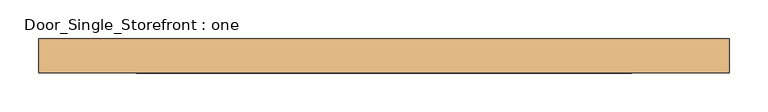
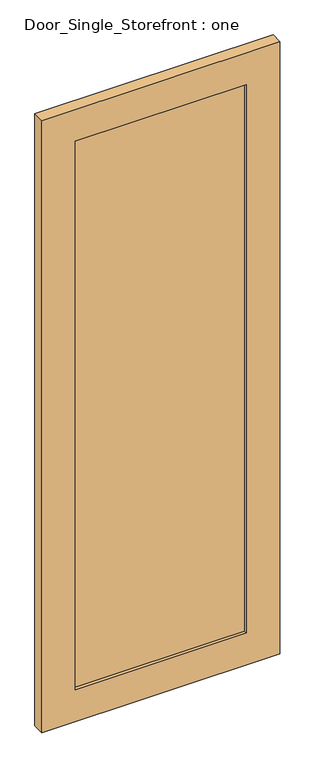
"""IFC4 building model written with IfcOpenShell, lengths in millimetres: door geometry, Door_Single_Storefront : one."""

import ifcopenshell
import ifcopenshell.guid

model = None  # the IFC model being written
_history = None  # IfcOwnerHistory: only IFC2X3 demands one
_inside = {}  # id of a spatial element -> (the spatial element, [elements in it])
_under = {}  # id of a project, library or spatial element -> (it, [spatial elements below it])
_declared = {}  # id of a project -> (the project, [libraries it declares])
_typed = {}  # id of a type object -> (the type object, [elements of that type])
_made_of = {}  # id of a material, layer set ... -> (it, [elements and type objects made of it])


def new_model(schema):
    """Start an empty IFC model of exactly this schema.

    Asked for "IFC4X3", IfcOpenShell would pick the latest addendum, in which some entities
    have other attributes; the version numbers below select the first issue.
    IFC2X3 requires an IfcOwnerHistory on every rooted entity: one is made here for all.
    """
    global model, _history
    if schema == "IFC4X3":
        model = ifcopenshell.file(schema_version=(4, 3, 0, 0))
    else:
        model = ifcopenshell.file(schema=schema)
    _inside.clear()
    _under.clear()
    _declared.clear()
    _typed.clear()
    _made_of.clear()
    _history = None
    if model.schema == "IFC2X3":
        org = make("IfcOrganization", Name="unknown")
        user = make(
            "IfcPersonAndOrganization",
            ThePerson=make("IfcPerson", FamilyName="unknown"),
            TheOrganization=org,
        )
        app = make(
            "IfcApplication",
            ApplicationDeveloper=org,
            Version="unknown",
            ApplicationFullName="unknown",
            ApplicationIdentifier="unknown",
        )
        _history = make(
            "IfcOwnerHistory",
            OwningUser=user,
            OwningApplication=app,
            ChangeAction="ADDED",
            CreationDate=0,
        )
    return model


def make(cls, **values):
    """One entity of the class cls with the attributes given. An attribute that is None is left unset."""
    return model.create_entity(
        cls, **{name: value for name, value in values.items() if value is not None}
    )


def rooted(cls, **values):
    """An entity with a GlobalId (a new one), such as an element, a storey or a relation."""
    return make(cls, GlobalId=ifcopenshell.guid.new(), OwnerHistory=_history, **values)


def si_unit(unit_type, name, prefix=None):
    """IfcSIUnit, for example si_unit("LENGTHUNIT", "METRE", prefix="MILLI")."""
    return make("IfcSIUnit", UnitType=unit_type, Prefix=prefix, Name=name)


def assignment(units):
    """IfcUnitAssignment: the units of a project."""
    return None if units is None else make("IfcUnitAssignment", Units=units)


def point(xyz):
    """IfcCartesianPoint."""
    return None if xyz is None else make("IfcCartesianPoint", Coordinates=xyz)


def direction(xyz):
    """IfcDirection."""
    return None if xyz is None else make("IfcDirection", DirectionRatios=xyz)


def frame(location, z_axis=None, x_axis=None):
    """IfcAxis2Placement3D, a coordinate frame: its origin and axes. An axis left out is left unset."""
    return make(
        "IfcAxis2Placement3D",
        Location=point(location),
        Axis=direction(z_axis),
        RefDirection=direction(x_axis),
    )


def origin():
    """The frame at (0, 0, 0) with its axes left unset."""
    return frame((0.0, 0.0, 0.0))


def place(relative_to, where):
    """IfcLocalPlacement: puts the frame where relative to a parent placement (None: the world)."""
    return make(
        "IfcLocalPlacement", PlacementRelTo=relative_to, RelativePlacement=where
    )


def context(
    kind, dimensions, precision=None, world=None, true_north=None, identifier=None
):
    """IfcGeometricRepresentationContext, for example the 3D "Model" context."""
    return make(
        "IfcGeometricRepresentationContext",
        ContextIdentifier=identifier,
        ContextType=kind,
        CoordinateSpaceDimension=dimensions,
        Precision=precision,
        WorldCoordinateSystem=world,
        TrueNorth=true_north,
    )


def project(units=None, contexts=None):
    """IfcProject with its units and contexts."""
    return rooted(
        "IfcProject",
        Name="project",
        RepresentationContexts=contexts,
        UnitsInContext=assignment(units),
    )


def spatial(cls, under=None, at=None, **own):
    """A site, building, storey or space (cls), placed at a placement, below another one or the project."""
    s = rooted(cls, ObjectPlacement=at, **own)
    if under is not None:
        _under.setdefault(under.id(), (under, []))[1].append(s)
    return s


def polyline(points):
    """IfcPolyline through the points."""
    return make("IfcPolyline", Points=[point(p) for p in points])


def outline(outer, holes=None, kind="AREA"):
    """IfcArbitraryClosedProfileDef: a profile drawn as a closed curve; with holes, ...WithVoids."""
    if holes is None:
        return make("IfcArbitraryClosedProfileDef", ProfileType=kind, OuterCurve=outer)
    return make(
        "IfcArbitraryProfileDefWithVoids",
        ProfileType=kind,
        OuterCurve=outer,
        InnerCurves=holes,
    )


def extrude(swept, where, along, depth):
    """IfcExtrudedAreaSolid: the profile swept, set in the frame where, extruded along a direction by depth."""
    return make(
        "IfcExtrudedAreaSolid",
        SweptArea=swept,
        Position=where,
        ExtrudedDirection=direction(along),
        Depth=depth,
    )


def shape(context_of_items, identifier, shape_type, items):
    """IfcShapeRepresentation: the items that make up one representation, for example the "Body"."""
    return make(
        "IfcShapeRepresentation",
        ContextOfItems=context_of_items,
        RepresentationIdentifier=identifier,
        RepresentationType=shape_type,
        Items=items,
    )


def source(mapping_origin, context_of_items, identifier, shape_type, items):
    """IfcRepresentationMap: a shape defined once, which mapped items show again and again."""
    return make(
        "IfcRepresentationMap",
        MappingOrigin=mapping_origin,
        MappedRepresentation=shape(context_of_items, identifier, shape_type, items),
    )


def transform(
    local_origin,
    x_axis=None,
    y_axis=None,
    z_axis=None,
    scale=None,
    scale2=None,
    scale3=None,
    uniform=True,
):
    """IfcCartesianTransformationOperator3D, or its non-uniform kind. x_axis, y_axis, z_axis: its Axis1, 2, 3."""
    if uniform:
        return make(
            "IfcCartesianTransformationOperator3D",
            Axis1=direction(x_axis),
            Axis2=direction(y_axis),
            LocalOrigin=point(local_origin),
            Scale=scale,
            Axis3=direction(z_axis),
        )
    return make(
        "IfcCartesianTransformationOperator3DnonUniform",
        Axis1=direction(x_axis),
        Axis2=direction(y_axis),
        LocalOrigin=point(local_origin),
        Scale=scale,
        Axis3=direction(z_axis),
        Scale2=scale2,
        Scale3=scale3,
    )


def mapped(mapping_source, mapping_target):
    """IfcMappedItem: shows the shape of a source again, moved by a transform."""
    return make(
        "IfcMappedItem", MappingSource=mapping_source, MappingTarget=mapping_target
    )


def made_of(thing, what):
    """Note that an element or type object is made of a material, layer set ...; save() writes the relation."""
    if what is not None:
        _made_of.setdefault(what.id(), (what, []))[1].append(thing)
    return thing


def element(
    cls,
    number,
    at=None,
    inside=None,
    cuts=None,
    type_object=None,
    material=None,
    context=None,
    identifier="Body",
    shape_type=None,
    held_by="IfcProductDefinitionShape",
    body=None,
    shapes=None,
    **own,
):
    """One element of the class cls, such as IfcWall. Its Tag is "e" and its number.

    at: its placement. inside: the storey or other place that contains it. cuts: it is an
    opening in that element (IfcRelVoidsElement). A single representation is given by context,
    identifier, shape_type and body (its items); several are given by shapes. held_by: the class
    of the entity that holds the representations. save() writes the other relations.
    """
    e = rooted(cls, Tag="e%d" % number, ObjectPlacement=at, **own)
    if body is not None:
        shapes = [shape(context, identifier, shape_type, body)]
    if shapes is not None:
        e.Representation = make(held_by, Representations=shapes)
    if inside is not None:
        _inside.setdefault(inside.id(), (inside, []))[1].append(e)
    if cuts is not None:
        rooted(
            "IfcRelVoidsElement", RelatingBuildingElement=cuts, RelatedOpeningElement=e
        )
    if type_object is not None:
        _typed.setdefault(type_object.id(), (type_object, []))[1].append(e)
    return made_of(e, material)


def aggregate(whole, parts):
    """IfcRelAggregates: a whole, such as a stair, and the parts it consists of."""
    return rooted("IfcRelAggregates", RelatingObject=whole, RelatedObjects=parts)


def save(model, path):
    """Write the relations noted so far, then the file.

    IfcRelAggregates (storeys below a building ...), IfcRelContainedInSpatialStructure (elements
    in a storey), IfcRelDefinesByType, IfcRelAssociatesMaterial and IfcRelDeclares: one each for
    every whole, place, type object, material and project.
    """
    for whole, parts in _under.values():
        aggregate(whole, parts)
    for where, things in _inside.values():
        rooted(
            "IfcRelContainedInSpatialStructure",
            RelatedElements=things,
            RelatingStructure=where,
        )
    for kind, things in _typed.values():
        rooted("IfcRelDefinesByType", RelatedObjects=things, RelatingType=kind)
    for what, things in _made_of.values():
        rooted("IfcRelAssociatesMaterial", RelatedObjects=things, RelatingMaterial=what)
    for by, libraries in _declared.values():
        rooted("IfcRelDeclares", RelatingContext=by, RelatedDefinitions=libraries)
    model.write(path)


def door_single_storefront_one_af52fb56(model_context):
    return source(origin(), model_context, "Body", "SweptSolid", [
        extrude(outline(polyline([(321.46875, -6.35), (-321.46875, -6.35), (-321.46875, 12.7), (321.46875, 12.7), (321.46875, -6.35)])), frame((0.0, 0.0, 127.0), z_axis=(0.0, 0.0, 1.0), x_axis=(1.0, 0.0, 0.0)), (0.0, 0.0, 1.0), 2184.4),
        extrude(outline(polyline([(2438.4, -448.46875), (0.0, -448.46875), (0.0, 448.46875), (2438.4, 448.46875), (2438.4, -448.46875)]), holes=[polyline([(127.0, 321.46875), (127.0, -321.46875), (2311.4, -321.46875), (2311.4, 321.46875), (127.0, 321.46875)])]), frame((0.0, -19.05, 0.0), z_axis=(0.0, 1.0, 0.0), x_axis=(0.0, 0.0, 1.0)), (0.0, 0.0, 1.0), 44.45),
    ])


if __name__ == "__main__":
    model = new_model("IFC4")
    model_context = context("Model", 3, world=origin())
    ifc_project = project(units=[si_unit("LENGTHUNIT", "METRE", prefix="MILLI")], contexts=[model_context])
    site = spatial("IfcSite", under=ifc_project)
    building = spatial("IfcBuilding", under=site)
    placement = place(None, origin())
    door_single_storefront_one_shape = door_single_storefront_one_af52fb56(model_context)
    element("IfcDoor", 1, ObjectType="Door_Single_Storefront : one", at=placement, inside=building, context=model_context, shape_type="MappedRepresentation", body=[
        mapped(door_single_storefront_one_shape, transform((0.0, 0.0, 0.0), x_axis=(1.0, 0.0, 0.0), y_axis=(0.0, 1.0, 0.0), z_axis=(0.0, 0.0, 1.0))),
    ])
    save(model, "model.ifc")

# Revit data of these elements
# Type "Door_Single_Storefront : one"
#   Type Mark = "27"
#   Analytic Construction = "<None>"
#   Stile_Width = 0' - 5"
#   Door_Thickness = 0' - 1 3/4"
#   Door_Offset = 0' - 1"
#   Glass_Material = SAFETY GLAZING
#   Frame_Material = INTERIOR GRADE ALUMINUM STOREFRONT W/ SAFETY GLAZING
#   Function = (empty or 0)
# Element 1 (IfcDoor, "Door_Single_Storefront : one")
#   Materials on its faces: "INTERIOR GRADE ALUMINUM STOREFRONT W/ SAFETY GLAZING", "SAFETY GLAZING"
# Materials
#   "SAFETY GLAZING": class "Glass", colour RGB 142 168 196, transparency 0.75, Description = "Soda Lime Glass", Cost = 0
#   "INTERIOR GRADE ALUMINUM STOREFRONT W/ SAFETY GLAZING": class "Metal", colour RGB 226 226 226, transparency 0, Description = "Aluminum 6061", Cost = 0
